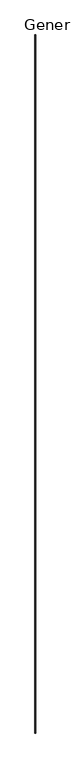
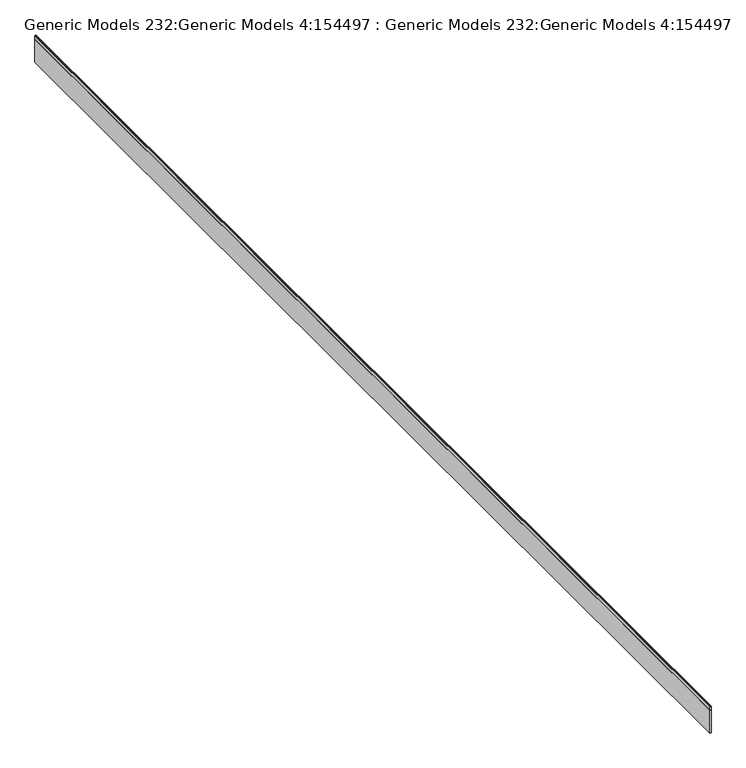
"""IFC4 building model written with IfcOpenShell, lengths in millimetres: proxy geometry, Generic Models 232:Generic Models 4:154497 : Generic Models 232:Generic Models 4:154497."""

import ifcopenshell
import ifcopenshell.guid

model = None  # the IFC model being written
_history = None  # IfcOwnerHistory: only IFC2X3 demands one
_inside = {}  # id of a spatial element -> (the spatial element, [elements in it])
_under = {}  # id of a project, library or spatial element -> (it, [spatial elements below it])
_declared = {}  # id of a project -> (the project, [libraries it declares])
_typed = {}  # id of a type object -> (the type object, [elements of that type])
_made_of = {}  # id of a material, layer set ... -> (it, [elements and type objects made of it])


def new_model(schema):
    """Start an empty IFC model of exactly this schema.

    Asked for "IFC4X3", IfcOpenShell would pick the latest addendum, in which some entities
    have other attributes; the version numbers below select the first issue.
    IFC2X3 requires an IfcOwnerHistory on every rooted entity: one is made here for all.
    """
    global model, _history
    if schema == "IFC4X3":
        model = ifcopenshell.file(schema_version=(4, 3, 0, 0))
    else:
        model = ifcopenshell.file(schema=schema)
    _inside.clear()
    _under.clear()
    _declared.clear()
    _typed.clear()
    _made_of.clear()
    _history = None
    if model.schema == "IFC2X3":
        org = make("IfcOrganization", Name="unknown")
        user = make(
            "IfcPersonAndOrganization",
            ThePerson=make("IfcPerson", FamilyName="unknown"),
            TheOrganization=org,
        )
        app = make(
            "IfcApplication",
            ApplicationDeveloper=org,
            Version="unknown",
            ApplicationFullName="unknown",
            ApplicationIdentifier="unknown",
        )
        _history = make(
            "IfcOwnerHistory",
            OwningUser=user,
            OwningApplication=app,
            ChangeAction="ADDED",
            CreationDate=0,
        )
    return model


def make(cls, **values):
    """One entity of the class cls with the attributes given. An attribute that is None is left unset."""
    return model.create_entity(
        cls, **{name: value for name, value in values.items() if value is not None}
    )


def rooted(cls, **values):
    """An entity with a GlobalId (a new one), such as an element, a storey or a relation."""
    return make(cls, GlobalId=ifcopenshell.guid.new(), OwnerHistory=_history, **values)


def si_unit(unit_type, name, prefix=None):
    """IfcSIUnit, for example si_unit("LENGTHUNIT", "METRE", prefix="MILLI")."""
    return make("IfcSIUnit", UnitType=unit_type, Prefix=prefix, Name=name)


def assignment(units):
    """IfcUnitAssignment: the units of a project."""
    return None if units is None else make("IfcUnitAssignment", Units=units)


def point(xyz):
    """IfcCartesianPoint."""
    return None if xyz is None else make("IfcCartesianPoint", Coordinates=xyz)


def direction(xyz):
    """IfcDirection."""
    return None if xyz is None else make("IfcDirection", DirectionRatios=xyz)


def frame(location, z_axis=None, x_axis=None):
    """IfcAxis2Placement3D, a coordinate frame: its origin and axes. An axis left out is left unset."""
    return make(
        "IfcAxis2Placement3D",
        Location=point(location),
        Axis=direction(z_axis),
        RefDirection=direction(x_axis),
    )


def origin():
    """The frame at (0, 0, 0) with its axes left unset."""
    return frame((0.0, 0.0, 0.0))


def place(relative_to, where):
    """IfcLocalPlacement: puts the frame where relative to a parent placement (None: the world)."""
    return make(
        "IfcLocalPlacement", PlacementRelTo=relative_to, RelativePlacement=where
    )


def context(
    kind, dimensions, precision=None, world=None, true_north=None, identifier=None
):
    """IfcGeometricRepresentationContext, for example the 3D "Model" context."""
    return make(
        "IfcGeometricRepresentationContext",
        ContextIdentifier=identifier,
        ContextType=kind,
        CoordinateSpaceDimension=dimensions,
        Precision=precision,
        WorldCoordinateSystem=world,
        TrueNorth=true_north,
    )


def project(units=None, contexts=None):
    """IfcProject with its units and contexts."""
    return rooted(
        "IfcProject",
        Name="project",
        RepresentationContexts=contexts,
        UnitsInContext=assignment(units),
    )


def spatial(cls, under=None, at=None, **own):
    """A site, building, storey or space (cls), placed at a placement, below another one or the project."""
    s = rooted(cls, ObjectPlacement=at, **own)
    if under is not None:
        _under.setdefault(under.id(), (under, []))[1].append(s)
    return s


def polyline(points):
    """IfcPolyline through the points."""
    return make("IfcPolyline", Points=[point(p) for p in points])


def outline(outer, holes=None, kind="AREA"):
    """IfcArbitraryClosedProfileDef: a profile drawn as a closed curve; with holes, ...WithVoids."""
    if holes is None:
        return make("IfcArbitraryClosedProfileDef", ProfileType=kind, OuterCurve=outer)
    return make(
        "IfcArbitraryProfileDefWithVoids",
        ProfileType=kind,
        OuterCurve=outer,
        InnerCurves=holes,
    )


def extrude(swept, where, along, depth):
    """IfcExtrudedAreaSolid: the profile swept, set in the frame where, extruded along a direction by depth."""
    return make(
        "IfcExtrudedAreaSolid",
        SweptArea=swept,
        Position=where,
        ExtrudedDirection=direction(along),
        Depth=depth,
    )


def shape(context_of_items, identifier, shape_type, items):
    """IfcShapeRepresentation: the items that make up one representation, for example the "Body"."""
    return make(
        "IfcShapeRepresentation",
        ContextOfItems=context_of_items,
        RepresentationIdentifier=identifier,
        RepresentationType=shape_type,
        Items=items,
    )


def source(mapping_origin, context_of_items, identifier, shape_type, items):
    """IfcRepresentationMap: a shape defined once, which mapped items show again and again."""
    return make(
        "IfcRepresentationMap",
        MappingOrigin=mapping_origin,
        MappedRepresentation=shape(context_of_items, identifier, shape_type, items),
    )


def transform(
    local_origin,
    x_axis=None,
    y_axis=None,
    z_axis=None,
    scale=None,
    scale2=None,
    scale3=None,
    uniform=True,
):
    """IfcCartesianTransformationOperator3D, or its non-uniform kind. x_axis, y_axis, z_axis: its Axis1, 2, 3."""
    if uniform:
        return make(
            "IfcCartesianTransformationOperator3D",
            Axis1=direction(x_axis),
            Axis2=direction(y_axis),
            LocalOrigin=point(local_origin),
            Scale=scale,
            Axis3=direction(z_axis),
        )
    return make(
        "IfcCartesianTransformationOperator3DnonUniform",
        Axis1=direction(x_axis),
        Axis2=direction(y_axis),
        LocalOrigin=point(local_origin),
        Scale=scale,
        Axis3=direction(z_axis),
        Scale2=scale2,
        Scale3=scale3,
    )


def mapped(mapping_source, mapping_target):
    """IfcMappedItem: shows the shape of a source again, moved by a transform."""
    return make(
        "IfcMappedItem", MappingSource=mapping_source, MappingTarget=mapping_target
    )


def made_of(thing, what):
    """Note that an element or type object is made of a material, layer set ...; save() writes the relation."""
    if what is not None:
        _made_of.setdefault(what.id(), (what, []))[1].append(thing)
    return thing


def element(
    cls,
    number,
    at=None,
    inside=None,
    cuts=None,
    type_object=None,
    material=None,
    context=None,
    identifier="Body",
    shape_type=None,
    held_by="IfcProductDefinitionShape",
    body=None,
    shapes=None,
    **own,
):
    """One element of the class cls, such as IfcWall. Its Tag is "e" and its number.

    at: its placement. inside: the storey or other place that contains it. cuts: it is an
    opening in that element (IfcRelVoidsElement). A single representation is given by context,
    identifier, shape_type and body (its items); several are given by shapes. held_by: the class
    of the entity that holds the representations. save() writes the other relations.
    """
    e = rooted(cls, Tag="e%d" % number, ObjectPlacement=at, **own)
    if body is not None:
        shapes = [shape(context, identifier, shape_type, body)]
    if shapes is not None:
        e.Representation = make(held_by, Representations=shapes)
    if inside is not None:
        _inside.setdefault(inside.id(), (inside, []))[1].append(e)
    if cuts is not None:
        rooted(
            "IfcRelVoidsElement", RelatingBuildingElement=cuts, RelatedOpeningElement=e
        )
    if type_object is not None:
        _typed.setdefault(type_object.id(), (type_object, []))[1].append(e)
    return made_of(e, material)


def aggregate(whole, parts):
    """IfcRelAggregates: a whole, such as a stair, and the parts it consists of."""
    return rooted("IfcRelAggregates", RelatingObject=whole, RelatedObjects=parts)


def save(model, path):
    """Write the relations noted so far, then the file.

    IfcRelAggregates (storeys below a building ...), IfcRelContainedInSpatialStructure (elements
    in a storey), IfcRelDefinesByType, IfcRelAssociatesMaterial and IfcRelDeclares: one each for
    every whole, place, type object, material and project.
    """
    for whole, parts in _under.values():
        aggregate(whole, parts)
    for where, things in _inside.values():
        rooted(
            "IfcRelContainedInSpatialStructure",
            RelatedElements=things,
            RelatingStructure=where,
        )
    for kind, things in _typed.values():
        rooted("IfcRelDefinesByType", RelatedObjects=things, RelatingType=kind)
    for what, things in _made_of.values():
        rooted("IfcRelAssociatesMaterial", RelatedObjects=things, RelatingMaterial=what)
    for by, libraries in _declared.values():
        rooted("IfcRelDeclares", RelatingContext=by, RelatedDefinitions=libraries)
    model.write(path)


def generic_models_232_generic_models_4_154497_generic_models_00dc09d8(model_context):
    return source(origin(), model_context, "Body", "SweptSolid", [
        extrude(outline(polyline([(1630.9443998, 11968.8025207), (1630.9443998, -6674.7974793), (1611.8943998, -6674.7974793), (1611.8943998, 11968.8025207), (1630.9443998, 11968.8025207)])), frame((0.0, 0.0, 2952.5528454), z_axis=(0.0, 0.0, 1.0), x_axis=(1.0, 0.0, 0.0)), (0.0, 0.0, 1.0), 384.6166708),
        extrude(outline(polyline([(3394.7606677, 1611.8943998), (3333.5528454, 1611.8943998), (3333.5528454, 1617.1517305), (3341.3676788, 1617.1517305), (3341.3676788, 1625.5244367), (3333.5528454, 1625.5244367), (3333.5528454, 1630.9443998), (3394.7606677, 1630.9443998), (3394.7606677, 1624.5943998), (3404.0395159, 1624.5943998), (3404.0395159, 1618.2443998), (3394.7606677, 1618.2443998), (3394.7606677, 1611.8943998)])), frame((0.0, -6674.7974793, 0.0), z_axis=(0.0, 1.0, 0.0), x_axis=(0.0, 0.0, 1.0)), (0.0, 0.0, 1.0), 18643.6),
    ])


if __name__ == "__main__":
    model = new_model("IFC4")
    model_context = context("Model", 3, world=origin())
    ifc_project = project(units=[si_unit("LENGTHUNIT", "METRE", prefix="MILLI")], contexts=[model_context])
    site = spatial("IfcSite", under=ifc_project)
    building = spatial("IfcBuilding", under=site)
    placement = place(None, origin())
    generic_models_232_generic_models_4_154497_generic_models_shape = generic_models_232_generic_models_4_154497_generic_models_00dc09d8(model_context)
    element("IfcBuildingElementProxy", 1, Name="Generic Models 232:Generic Models 4:154497 : Generic Models 232:Generic Models 4:154497", ObjectType="Generic Models 232:Generic Models 4:154497 : Generic Models 232:Generic Models 4:154497", at=placement, inside=building, context=model_context, shape_type="MappedRepresentation", body=[
        mapped(generic_models_232_generic_models_4_154497_generic_models_shape, transform((0.0, 0.0, 0.0), x_axis=(1.0, 0.0, 0.0), y_axis=(0.0, 1.0, 0.0), z_axis=(0.0, 0.0, 1.0))),
    ])
    save(model, "model.ifc")

# Revit data of these elements
# Type "Generic Models 232:Generic Models 4:154497 : Generic Models 232:Generic Models 4:154497"
#   NameOverride = "Generic Models 232:Generic Models 4:154497"
#   ObjectTypeOverride = "Generic Models 232:Generic Models 4"
#   Reference = "Generic Models 4"
#   Category = "Generic Models"
#   Tag = "154497"
# Element 1 (IfcBuildingElementProxy, "Generic Models 232:Generic Models 4:154497 : Generic Models 232:Generic Models 4:154497")
#   Materials on its faces: "_FIRE RETARDANT WOOD SIDING T.B.D 23315"
# Materials
#   "_FIRE RETARDANT WOOD SIDING T.B.D 23315": class "Unassigned", colour RGB 177 130 114, transparency 0
